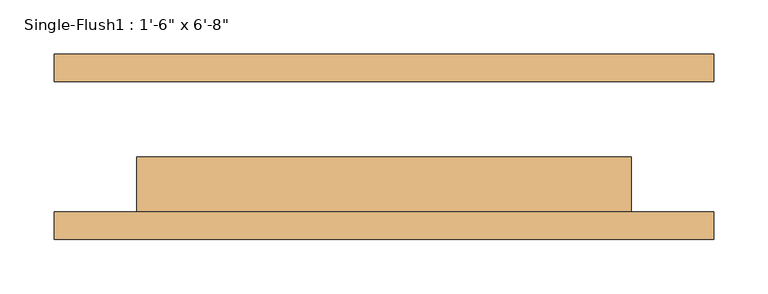
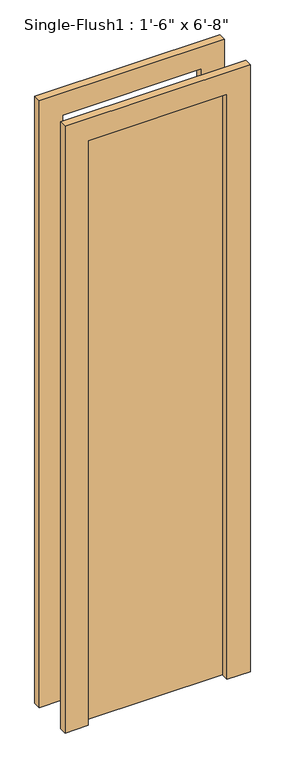
"""IFC4 building model written with IfcOpenShell, lengths in millimetres: door geometry."""

from ifc_helpers import new_model, si_unit, frame, origin, origin_with_axes, place, context, project, spatial, polyline, outline, extrude, source, transform, mapped, element, save


def door_8bf1a118(model_context):
    return source(origin(), model_context, "Body", "SweptSolid", [
        extrude(outline(polyline([(2108.2, -304.8), (0.0, -304.8), (0.0, -228.6), (2032.0, -228.6), (2032.0, 228.6), (0.0, 228.6), (0.0, 304.8), (2108.2, 304.8), (2108.2, -304.8)])), frame((0.0, -85.725, 0.0), z_axis=(0.0, 1.0, 0.0), x_axis=(0.0, 0.0, 1.0)), (0.0, 0.0, 1.0), 25.4),
        extrude(outline(polyline([(2108.2, 304.8), (2108.2, -304.8), (0.0, -304.8), (0.0, -228.6), (2032.0, -228.6), (2032.0, 228.6), (0.0, 228.6), (0.0, 304.8), (2108.2, 304.8)])), frame((0.0, 60.325, 0.0), z_axis=(0.0, 1.0, 0.0), x_axis=(0.0, 0.0, 1.0)), (0.0, 0.0, 1.0), 25.4),
        extrude(outline(polyline([(228.6, -9.525), (228.6, -60.325), (-228.6, -60.325), (-228.6, -9.525), (228.6, -9.525)])), origin_with_axes(), (0.0, 0.0, 1.0), 2032.0),
    ])


if __name__ == "__main__":
    model = new_model("IFC4")
    model_context = context("Model", 3, world=origin())
    ifc_project = project(units=[si_unit("LENGTHUNIT", "METRE", prefix="MILLI")], contexts=[model_context])
    site = spatial("IfcSite", under=ifc_project)
    building = spatial("IfcBuilding", under=site)
    placement = place(None, origin())
    door_shape = door_8bf1a118(model_context)
    element("IfcDoor", 1, ObjectType="Single-Flush1 : 1'-6\" x 6'-8\"", at=placement, inside=building, context=model_context, shape_type="MappedRepresentation", body=[
        mapped(door_shape, transform((0.0, 0.0, 0.0), x_axis=(1.0, 0.0, 0.0), y_axis=(0.0, 1.0, 0.0), z_axis=(0.0, 0.0, 1.0))),
    ])
    save(model, "model.ifc")

# Revit data of these elements
# Type "Single-Flush1 : 1'-6\" x 6'-8\""
#   Type Mark = "D5"
#   Construction Type Id = "MDOOR"
#   Assembly Code = "C1020"
#   Analytic Construction = "Metal"
#   Thickness = 0' - 2"
#   Heat Transfer Coefficient (U) = 3.7021 W/(m²·K)
#   Height = 6' - 8"
#   Trim Projection Ext = 0' - 1"
#   Trim Projection Int = 0' - 1"
#   Trim Width = 0' - 3"
#   Width = 1' - 6"
#   Door Material = Door - Panel
#   Frame Material = Door - Frame
#   Visual Light Transmittance = 0
#   Solar Heat Gain Coefficient = 0
#   Function = (empty or 0)
#   Wall Closure = (empty or 0)
# Element 1 (IfcDoor, "Single-Flush1 : 1'-6\" x 6'-8\"")
#   Materials on its faces: "Door - Frame", "Door - Panel"
# Materials
#   "Door - Panel": class "Wood", colour RGB 210 159 95, transparency 0, Cost = 0
#   "Door - Frame": class "Miscellaneous", colour RGB 118 70 51, transparency 0, Cost = 0
